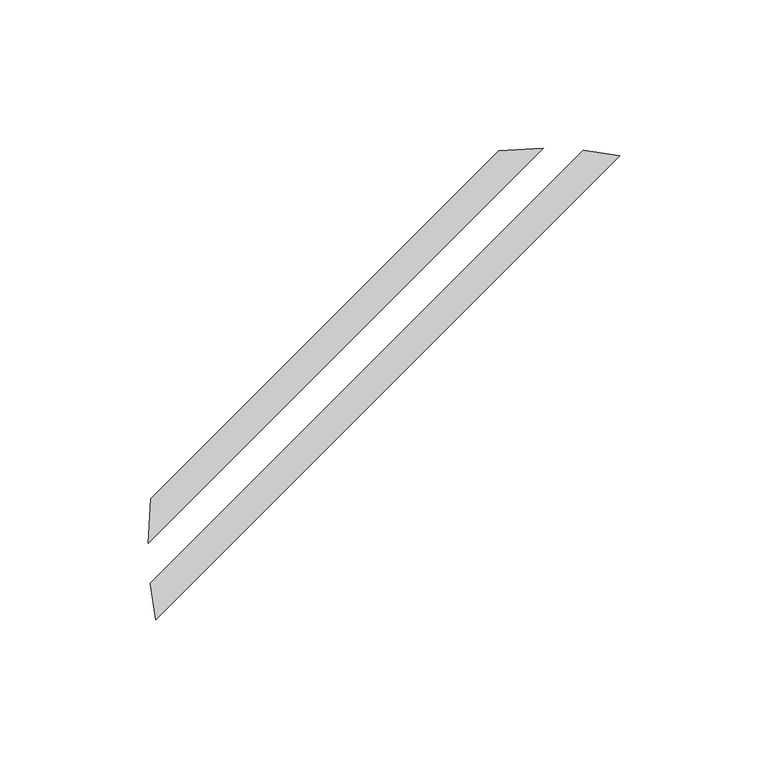
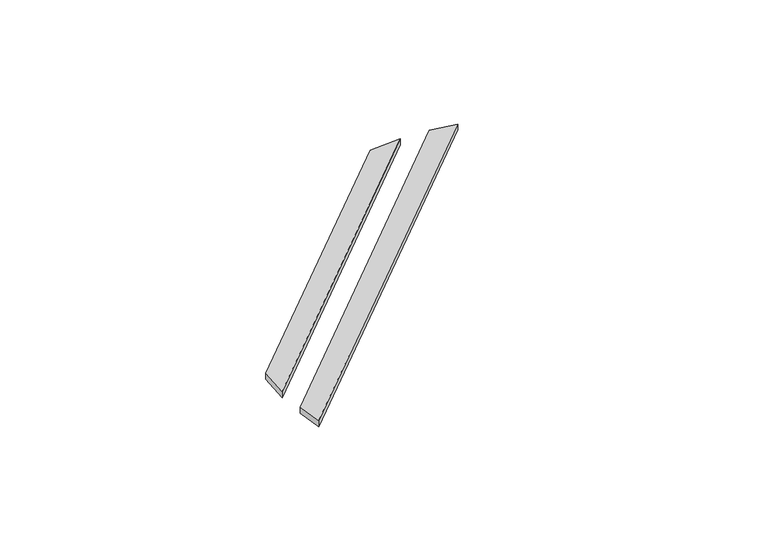
"""IFC4 building model written with IfcOpenShell, lengths in millimetres: proxy geometry, TSP Downlighter in Ceiling : TSP Downlighter in Ceiling."""

import ifcopenshell
import ifcopenshell.guid

model = None  # the IFC model being written
_history = None  # IfcOwnerHistory: only IFC2X3 demands one
_inside = {}  # id of a spatial element -> (the spatial element, [elements in it])
_under = {}  # id of a project, library or spatial element -> (it, [spatial elements below it])
_declared = {}  # id of a project -> (the project, [libraries it declares])
_typed = {}  # id of a type object -> (the type object, [elements of that type])
_made_of = {}  # id of a material, layer set ... -> (it, [elements and type objects made of it])


def new_model(schema):
    """Start an empty IFC model of exactly this schema.

    Asked for "IFC4X3", IfcOpenShell would pick the latest addendum, in which some entities
    have other attributes; the version numbers below select the first issue.
    IFC2X3 requires an IfcOwnerHistory on every rooted entity: one is made here for all.
    """
    global model, _history
    if schema == "IFC4X3":
        model = ifcopenshell.file(schema_version=(4, 3, 0, 0))
    else:
        model = ifcopenshell.file(schema=schema)
    _inside.clear()
    _under.clear()
    _declared.clear()
    _typed.clear()
    _made_of.clear()
    _history = None
    if model.schema == "IFC2X3":
        org = make("IfcOrganization", Name="unknown")
        user = make(
            "IfcPersonAndOrganization",
            ThePerson=make("IfcPerson", FamilyName="unknown"),
            TheOrganization=org,
        )
        app = make(
            "IfcApplication",
            ApplicationDeveloper=org,
            Version="unknown",
            ApplicationFullName="unknown",
            ApplicationIdentifier="unknown",
        )
        _history = make(
            "IfcOwnerHistory",
            OwningUser=user,
            OwningApplication=app,
            ChangeAction="ADDED",
            CreationDate=0,
        )
    return model


def make(cls, **values):
    """One entity of the class cls with the attributes given. An attribute that is None is left unset."""
    return model.create_entity(
        cls, **{name: value for name, value in values.items() if value is not None}
    )


def rooted(cls, **values):
    """An entity with a GlobalId (a new one), such as an element, a storey or a relation."""
    return make(cls, GlobalId=ifcopenshell.guid.new(), OwnerHistory=_history, **values)


def si_unit(unit_type, name, prefix=None):
    """IfcSIUnit, for example si_unit("LENGTHUNIT", "METRE", prefix="MILLI")."""
    return make("IfcSIUnit", UnitType=unit_type, Prefix=prefix, Name=name)


def assignment(units):
    """IfcUnitAssignment: the units of a project."""
    return None if units is None else make("IfcUnitAssignment", Units=units)


def point(xyz):
    """IfcCartesianPoint."""
    return None if xyz is None else make("IfcCartesianPoint", Coordinates=xyz)


def direction(xyz):
    """IfcDirection."""
    return None if xyz is None else make("IfcDirection", DirectionRatios=xyz)


def frame(location, z_axis=None, x_axis=None):
    """IfcAxis2Placement3D, a coordinate frame: its origin and axes. An axis left out is left unset."""
    return make(
        "IfcAxis2Placement3D",
        Location=point(location),
        Axis=direction(z_axis),
        RefDirection=direction(x_axis),
    )


def frame_2d(location, x_axis=None):
    """IfcAxis2Placement2D, a coordinate frame in the plane: its origin and x axis."""
    return make(
        "IfcAxis2Placement2D", Location=point(location), RefDirection=direction(x_axis)
    )


def origin():
    """The frame at (0, 0, 0) with its axes left unset."""
    return frame((0.0, 0.0, 0.0))


def origin_with_axes():
    """The frame at (0, 0, 0) with the z axis (0, 0, 1) and the x axis (1, 0, 0) written out."""
    return frame((0.0, 0.0, 0.0), z_axis=(0.0, 0.0, 1.0), x_axis=(1.0, 0.0, 0.0))


def origin_2d():
    """The frame at (0, 0) in the plane with its x axis left unset."""
    return frame_2d((0.0, 0.0))


def place(relative_to, where):
    """IfcLocalPlacement: puts the frame where relative to a parent placement (None: the world)."""
    return make(
        "IfcLocalPlacement", PlacementRelTo=relative_to, RelativePlacement=where
    )


def context(
    kind, dimensions, precision=None, world=None, true_north=None, identifier=None
):
    """IfcGeometricRepresentationContext, for example the 3D "Model" context."""
    return make(
        "IfcGeometricRepresentationContext",
        ContextIdentifier=identifier,
        ContextType=kind,
        CoordinateSpaceDimension=dimensions,
        Precision=precision,
        WorldCoordinateSystem=world,
        TrueNorth=true_north,
    )


def project(units=None, contexts=None):
    """IfcProject with its units and contexts."""
    return rooted(
        "IfcProject",
        Name="project",
        RepresentationContexts=contexts,
        UnitsInContext=assignment(units),
    )


def spatial(cls, under=None, at=None, **own):
    """A site, building, storey or space (cls), placed at a placement, below another one or the project."""
    s = rooted(cls, ObjectPlacement=at, **own)
    if under is not None:
        _under.setdefault(under.id(), (under, []))[1].append(s)
    return s


def polyline(points):
    """IfcPolyline through the points."""
    return make("IfcPolyline", Points=[point(p) for p in points])


def circle_curve(where, radius):
    """IfcCircle in the frame where."""
    return make("IfcCircle", Position=where, Radius=radius)


def trimmed(basis, trim1, trim2, sense, master):
    """IfcTrimmedCurve: the piece of a basis curve between two trims."""
    return make(
        "IfcTrimmedCurve",
        BasisCurve=basis,
        Trim1=trim1,
        Trim2=trim2,
        SenseAgreement=sense,
        MasterRepresentation=master,
    )


def segment(curve, same_sense, transition):
    """IfcCompositeCurveSegment."""
    return make(
        "IfcCompositeCurveSegment",
        Transition=transition,
        SameSense=same_sense,
        ParentCurve=curve,
    )


def composite_curve(segments, self_intersect=None):
    """IfcCompositeCurve: segments joined end to end."""
    return make("IfcCompositeCurve", Segments=segments, SelfIntersect=self_intersect)


def outline(outer, holes=None, kind="AREA"):
    """IfcArbitraryClosedProfileDef: a profile drawn as a closed curve; with holes, ...WithVoids."""
    if holes is None:
        return make("IfcArbitraryClosedProfileDef", ProfileType=kind, OuterCurve=outer)
    return make(
        "IfcArbitraryProfileDefWithVoids",
        ProfileType=kind,
        OuterCurve=outer,
        InnerCurves=holes,
    )


def extrude(swept, where, along, depth):
    """IfcExtrudedAreaSolid: the profile swept, set in the frame where, extruded along a direction by depth."""
    return make(
        "IfcExtrudedAreaSolid",
        SweptArea=swept,
        Position=where,
        ExtrudedDirection=direction(along),
        Depth=depth,
    )


def shape(context_of_items, identifier, shape_type, items):
    """IfcShapeRepresentation: the items that make up one representation, for example the "Body"."""
    return make(
        "IfcShapeRepresentation",
        ContextOfItems=context_of_items,
        RepresentationIdentifier=identifier,
        RepresentationType=shape_type,
        Items=items,
    )


def source(mapping_origin, context_of_items, identifier, shape_type, items):
    """IfcRepresentationMap: a shape defined once, which mapped items show again and again."""
    return make(
        "IfcRepresentationMap",
        MappingOrigin=mapping_origin,
        MappedRepresentation=shape(context_of_items, identifier, shape_type, items),
    )


def transform(
    local_origin,
    x_axis=None,
    y_axis=None,
    z_axis=None,
    scale=None,
    scale2=None,
    scale3=None,
    uniform=True,
):
    """IfcCartesianTransformationOperator3D, or its non-uniform kind. x_axis, y_axis, z_axis: its Axis1, 2, 3."""
    if uniform:
        return make(
            "IfcCartesianTransformationOperator3D",
            Axis1=direction(x_axis),
            Axis2=direction(y_axis),
            LocalOrigin=point(local_origin),
            Scale=scale,
            Axis3=direction(z_axis),
        )
    return make(
        "IfcCartesianTransformationOperator3DnonUniform",
        Axis1=direction(x_axis),
        Axis2=direction(y_axis),
        LocalOrigin=point(local_origin),
        Scale=scale,
        Axis3=direction(z_axis),
        Scale2=scale2,
        Scale3=scale3,
    )


def mapped(mapping_source, mapping_target):
    """IfcMappedItem: shows the shape of a source again, moved by a transform."""
    return make(
        "IfcMappedItem", MappingSource=mapping_source, MappingTarget=mapping_target
    )


def made_of(thing, what):
    """Note that an element or type object is made of a material, layer set ...; save() writes the relation."""
    if what is not None:
        _made_of.setdefault(what.id(), (what, []))[1].append(thing)
    return thing


def element(
    cls,
    number,
    at=None,
    inside=None,
    cuts=None,
    type_object=None,
    material=None,
    context=None,
    identifier="Body",
    shape_type=None,
    held_by="IfcProductDefinitionShape",
    body=None,
    shapes=None,
    **own,
):
    """One element of the class cls, such as IfcWall. Its Tag is "e" and its number.

    at: its placement. inside: the storey or other place that contains it. cuts: it is an
    opening in that element (IfcRelVoidsElement). A single representation is given by context,
    identifier, shape_type and body (its items); several are given by shapes. held_by: the class
    of the entity that holds the representations. save() writes the other relations.
    """
    e = rooted(cls, Tag="e%d" % number, ObjectPlacement=at, **own)
    if body is not None:
        shapes = [shape(context, identifier, shape_type, body)]
    if shapes is not None:
        e.Representation = make(held_by, Representations=shapes)
    if inside is not None:
        _inside.setdefault(inside.id(), (inside, []))[1].append(e)
    if cuts is not None:
        rooted(
            "IfcRelVoidsElement", RelatingBuildingElement=cuts, RelatedOpeningElement=e
        )
    if type_object is not None:
        _typed.setdefault(type_object.id(), (type_object, []))[1].append(e)
    return made_of(e, material)


def aggregate(whole, parts):
    """IfcRelAggregates: a whole, such as a stair, and the parts it consists of."""
    return rooted("IfcRelAggregates", RelatingObject=whole, RelatedObjects=parts)


def save(model, path):
    """Write the relations noted so far, then the file.

    IfcRelAggregates (storeys below a building ...), IfcRelContainedInSpatialStructure (elements
    in a storey), IfcRelDefinesByType, IfcRelAssociatesMaterial and IfcRelDeclares: one each for
    every whole, place, type object, material and project.
    """
    for whole, parts in _under.values():
        aggregate(whole, parts)
    for where, things in _inside.values():
        rooted(
            "IfcRelContainedInSpatialStructure",
            RelatedElements=things,
            RelatingStructure=where,
        )
    for kind, things in _typed.values():
        rooted("IfcRelDefinesByType", RelatedObjects=things, RelatingType=kind)
    for what, things in _made_of.values():
        rooted("IfcRelAssociatesMaterial", RelatedObjects=things, RelatingMaterial=what)
    for by, libraries in _declared.values():
        rooted("IfcRelDeclares", RelatingContext=by, RelatedDefinitions=libraries)
    model.write(path)


def electrical_fixtures_f9291149(model_context):
    return source(origin(), model_context, "Body", "SweptSolid", [
        extrude(outline(composite_curve([segment(trimmed(circle_curve(origin_2d(), 133.3333333), [point((-14.987114, 132.4883549))], [point((0.0, 133.3333333))], False, "CARTESIAN"), True, "CONTINUOUS"), segment(polyline([(0.0, 133.3333333), (-133.3333333, 0.0)]), True, "CONTINUOUS"), segment(trimmed(circle_curve(origin_2d(), 133.3333333), [point((-133.3333333, 0.0))], [point((-132.4883549, 14.987114))], False, "CARTESIAN"), True, "CONTINUOUS"), segment(polyline([(-132.4883549, 14.987114), (-14.987114, 132.4883549)]), True, "CONTINUOUS")], self_intersect=False)), origin_with_axes(), (0.0, 0.0, 1.0), 3.0),
        extrude(outline(composite_curve([segment(trimmed(circle_curve(origin_2d(), 133.3333333), [point((13.46091, 132.6521077))], [point((25.7701848, 130.8192469))], False, "CARTESIAN"), True, "CONTINUOUS"), segment(polyline([(25.7701848, 130.8192469), (-130.8192469, -25.7701848)]), True, "CONTINUOUS"), segment(trimmed(circle_curve(origin_2d(), 133.3333333), [point((-130.8192469, -25.7701848))], [point((-132.6521077, -13.46091))], False, "CARTESIAN"), True, "CONTINUOUS"), segment(polyline([(-132.6521077, -13.46091), (13.46091, 132.6521077)]), True, "CONTINUOUS")], self_intersect=False)), origin_with_axes(), (0.0, 0.0, 1.0), 3.0),
    ])


if __name__ == "__main__":
    model = new_model("IFC4")
    model_context = context("Model", 3, world=origin())
    ifc_project = project(units=[si_unit("LENGTHUNIT", "METRE", prefix="MILLI")], contexts=[model_context])
    site = spatial("IfcSite", under=ifc_project)
    building = spatial("IfcBuilding", under=site)
    placement = place(None, origin())
    electrical_fixtures_shape = electrical_fixtures_f9291149(model_context)
    element("IfcBuildingElementProxy", 1, Name="TSP Downlighter in Ceiling : TSP Downlighter in Ceiling", ObjectType="TSP Downlighter in Ceiling : TSP Downlighter in Ceiling", at=placement, inside=building, context=model_context, shape_type="MappedRepresentation", body=[
        mapped(electrical_fixtures_shape, transform((0.0, 0.0, 0.0), x_axis=(1.0, 0.0, 0.0), y_axis=(0.0, 1.0, 0.0), z_axis=(0.0, 0.0, 1.0))),
    ])
    save(model, "model.ifc")

# Revit data of these elements
# Type "TSP Downlighter in Ceiling : TSP Downlighter in Ceiling"
#   Model = "TSP_ELEC220DLCEIL"
#   Default Elevation = 0
# Element 1 (IfcBuildingElementProxy, "TSP Downlighter in Ceiling : TSP Downlighter in Ceiling")
#   Materials on its faces: "Plastic, Opaque Black"
# Materials
#   "Plastic, Opaque Black": class "Plastic", colour RGB 0 0 0, transparency 0.7, Description = "Plastic, generic, opaque black", Cost = 0
